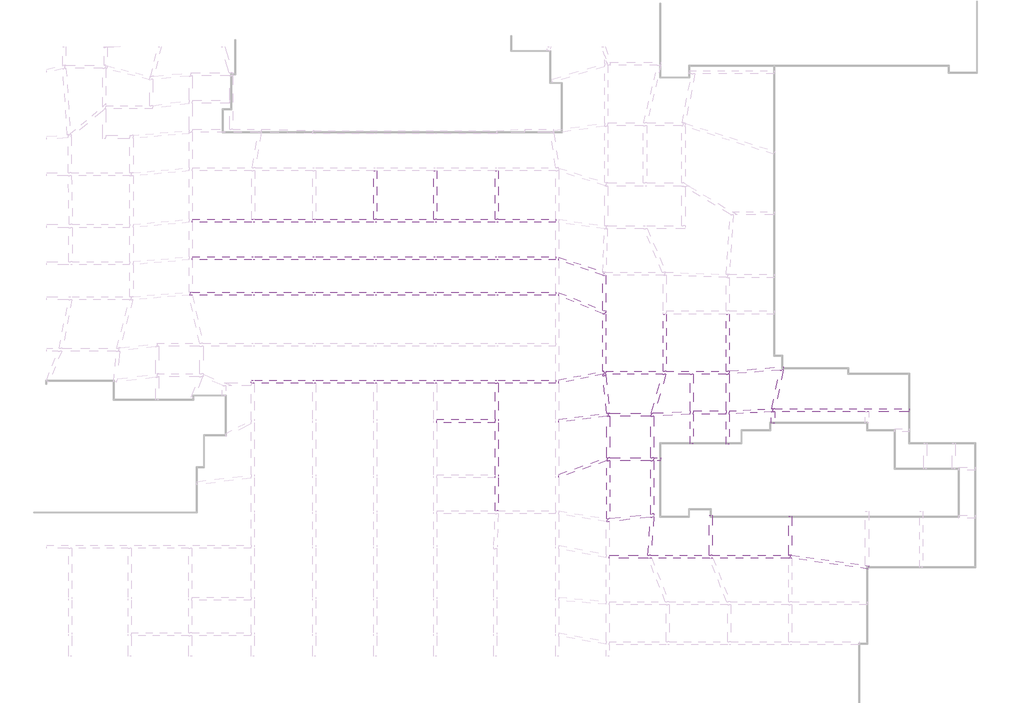
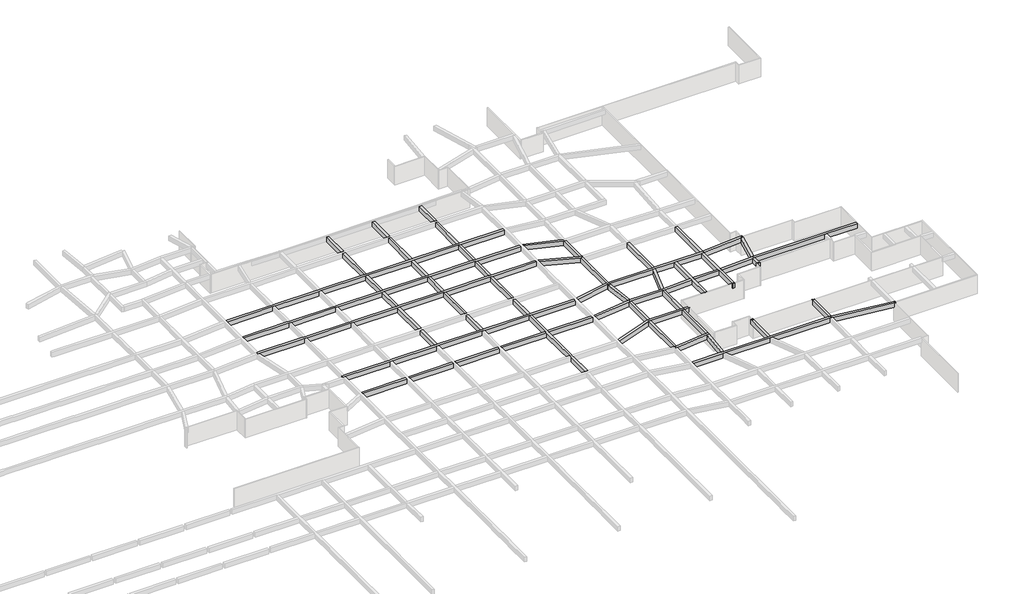
# One storey, part 40 of 45: 43 beams.
"""IFC4 building model written with IfcOpenShell, lengths in millimetres."""

from ifc_helpers import new_model, si_unit, frame, origin, place, context, project, spatial, polyline, outline, extrude, faceted_brep, element, save

model = new_model("IFC4")

# Units and contexts
model_context = context("Model", 3, world=origin())
ifc_project = project(units=[si_unit("LENGTHUNIT", "METRE", prefix="MILLI")], contexts=[model_context])

# Site, building, storey
site = spatial("IfcSite", under=ifc_project)
building = spatial("IfcBuilding", under=site)
storey = spatial("IfcBuildingStorey", under=building, Name="户型图", Elevation=0.0)

# Beams
placement = place(None, origin())
element("IfcBeam", 1, ObjectType="混凝土 - 矩形梁 : KL_beam", at=placement, inside=storey, context=model_context, shape_type="Brep", body=[
    faceted_brep([(24442.7166646, 44499.769125, 3300.0), (24442.7166646, 44899.769125, 3300.0), (17069.3873949, 44899.769125, 3300.0), (16669.3873949, 44899.769125, 3300.0), (9169.3873949, 44899.769125, 3300.0), (8769.3873949, 44899.769125, 3300.0), (1471.7652295, 44899.769125, 3300.0), (1071.7652295, 44899.769125, 3300.0), (-6328.2347705, 44899.769125, 3300.0), (-6728.2347705, 44899.769125, 3300.0), (-14137.8475592, 44899.769125, 3300.0), (-14537.8475592, 44899.769125, 3300.0), (-22164.0859234, 44899.769125, 3300.0), (-22164.0859234, 44499.769125, 3300.0), (-14537.8475592, 44499.769125, 3300.0), (-14137.8475592, 44499.769125, 3300.0), (-6728.2347705, 44499.769125, 3300.0), (-6328.2347705, 44499.769125, 3300.0), (1071.7652295, 44499.769125, 3300.0), (1471.7652295, 44499.769125, 3300.0), (8769.3873949, 44499.769125, 3300.0), (9169.3873949, 44499.769125, 3300.0), (16669.3873949, 44499.769125, 3300.0), (17069.3873949, 44499.769125, 3300.0), (24442.7166646, 44499.769125, 2500.0), (-22164.0859234, 44499.769125, 2500.0), (-14537.8475592, 44499.769125, 2500.0), (-14137.8475592, 44499.769125, 2500.0), (-6728.2347705, 44499.769125, 2500.0), (-6328.2347705, 44499.769125, 2500.0), (1071.7652295, 44499.769125, 2500.0), (1471.7652295, 44499.769125, 2500.0), (8769.3873949, 44499.769125, 2500.0), (9169.3873949, 44499.769125, 2500.0), (16669.3873949, 44499.769125, 2500.0), (17069.3873949, 44499.769125, 2500.0), (24442.7166646, 44899.769125, 2500.0), (-22164.0859234, 44899.769125, 2500.0), (-14537.8475592, 44899.769125, 2500.0), (-14137.8475592, 44899.769125, 2500.0), (-6728.2347705, 44899.769125, 2500.0), (-6328.2347705, 44899.769125, 2500.0), (1071.7652295, 44899.769125, 2500.0), (1471.7652295, 44899.769125, 2500.0), (8769.3873949, 44899.769125, 2500.0), (9169.3873949, 44899.769125, 2500.0), (16669.3873949, 44899.769125, 2500.0), (17069.3873949, 44899.769125, 2500.0)], [[[0, 1, 2, 3, 4, 5, 6, 7, 8, 9, 10, 11, 12, 13, 14, 15, 16, 17, 18, 19, 20, 21, 22, 23]], [[24, 0, 23, 22, 21, 20, 19, 18, 17, 16, 15, 14, 13, 25, 26, 27, 28, 29, 30, 31, 32, 33, 34, 35]], [[36, 24, 35, 34, 33, 32, 31, 30, 29, 28, 27, 26, 25, 37, 38, 39, 40, 41, 42, 43, 44, 45, 46, 47]], [[1, 36, 47, 46, 45, 44, 43, 42, 41, 40, 39, 38, 37, 12, 11, 10, 9, 8, 7, 6, 5, 4, 3, 2]], [[1, 0, 24, 36]], [[13, 12, 37, 25]]]),
])
element("IfcBeam", 2, ObjectType="混凝土 - 矩形梁 : KL_beam", at=placement, inside=storey, context=model_context, shape_type="Brep", body=[
    faceted_brep([(24442.7166646, 39701.2747355, 3300.0), (24442.7166646, 40101.2747355, 3300.0), (17069.3873949, 40101.2747355, 3300.0), (16669.3873949, 40101.2747355, 3300.0), (9169.3873949, 40101.2747355, 3300.0), (8769.3873949, 40101.2747355, 3300.0), (1471.7652295, 40101.2747355, 3300.0), (1071.7652295, 40101.2747355, 3300.0), (-6328.2347705, 40101.2747355, 3300.0), (-6728.2347705, 40101.2747355, 3300.0), (-14137.8475592, 40101.2747355, 3300.0), (-14537.8475592, 40101.2747355, 3300.0), (-22164.0859234, 40101.2747355, 3300.0), (-22164.0859234, 39701.2747355, 3300.0), (-14537.8475592, 39701.2747355, 3300.0), (-14137.8475592, 39701.2747355, 3300.0), (-6728.2347705, 39701.2747355, 3300.0), (-6328.2347705, 39701.2747355, 3300.0), (1071.7652295, 39701.2747355, 3300.0), (1471.7652295, 39701.2747355, 3300.0), (8769.3873949, 39701.2747355, 3300.0), (9169.3873949, 39701.2747355, 3300.0), (16669.3873949, 39701.2747355, 3300.0), (17069.3873949, 39701.2747355, 3300.0), (24442.7166646, 39701.2747355, 2500.0), (-22164.0859234, 39701.2747355, 2500.0), (-14537.8475592, 39701.2747355, 2500.0), (-14137.8475592, 39701.2747355, 2500.0), (-6728.2347705, 39701.2747355, 2500.0), (-6328.2347705, 39701.2747355, 2500.0), (1071.7652295, 39701.2747355, 2500.0), (1471.7652295, 39701.2747355, 2500.0), (8769.3873949, 39701.2747355, 2500.0), (9169.3873949, 39701.2747355, 2500.0), (16669.3873949, 39701.2747355, 2500.0), (17069.3873949, 39701.2747355, 2500.0), (24442.7166646, 40101.2747355, 2500.0), (-22164.0859234, 40101.2747355, 2500.0), (-14537.8475592, 40101.2747355, 2500.0), (-14137.8475592, 40101.2747355, 2500.0), (-6728.2347705, 40101.2747355, 2500.0), (-6328.2347705, 40101.2747355, 2500.0), (1071.7652295, 40101.2747355, 2500.0), (1471.7652295, 40101.2747355, 2500.0), (8769.3873949, 40101.2747355, 2500.0), (9169.3873949, 40101.2747355, 2500.0), (16669.3873949, 40101.2747355, 2500.0), (17069.3873949, 40101.2747355, 2500.0)], [[[0, 1, 2, 3, 4, 5, 6, 7, 8, 9, 10, 11, 12, 13, 14, 15, 16, 17, 18, 19, 20, 21, 22, 23]], [[24, 0, 23, 22, 21, 20, 19, 18, 17, 16, 15, 14, 13, 25, 26, 27, 28, 29, 30, 31, 32, 33, 34, 35]], [[36, 24, 35, 34, 33, 32, 31, 30, 29, 28, 27, 26, 25, 37, 38, 39, 40, 41, 42, 43, 44, 45, 46, 47]], [[1, 36, 47, 46, 45, 44, 43, 42, 41, 40, 39, 38, 37, 12, 11, 10, 9, 8, 7, 6, 5, 4, 3, 2]], [[1, 0, 24, 36]], [[13, 12, 37, 25]]]),
])
element("IfcBeam", 3, ObjectType="混凝土 - 矩形梁 : KL_beam", at=placement, inside=storey, context=model_context, shape_type="Brep", body=[
    faceted_brep([(-22423.5665565, 35573.301237, 3300.0), (-22407.6688706, 35173.301237, 3300.0), (-22167.3046288, 35173.301237, 3300.0), (-14537.8475592, 35173.301237, 3300.0), (-14137.8475592, 35173.301237, 3300.0), (-6728.2347705, 35173.301237, 3300.0), (-6328.2347705, 35173.301237, 3300.0), (1071.7652295, 35173.301237, 3300.0), (1471.7652295, 35173.301237, 3300.0), (8769.3873949, 35173.301237, 3300.0), (9169.3873949, 35173.301237, 3300.0), (16669.3873949, 35173.301237, 3300.0), (17069.3873949, 35173.301237, 3300.0), (24442.7166646, 35173.301237, 3300.0), (24442.7166646, 35573.301237, 3300.0), (17069.3873949, 35573.301237, 3300.0), (16669.3873949, 35573.301237, 3300.0), (9169.3873949, 35573.301237, 3300.0), (8769.3873949, 35573.301237, 3300.0), (1471.7652295, 35573.301237, 3300.0), (1071.7652295, 35573.301237, 3300.0), (-6328.2347705, 35573.301237, 3300.0), (-6728.2347705, 35573.301237, 3300.0), (-14137.8475592, 35573.301237, 3300.0), (-14537.8475592, 35573.301237, 3300.0), (-22164.0859234, 35573.301237, 3300.0), (-22407.6688706, 35173.301237, 2500.0), (-22167.3046288, 35173.301237, 2500.0), (-14537.8475592, 35173.301237, 2500.0), (-14137.8475592, 35173.301237, 2500.0), (-6728.2347705, 35173.301237, 2500.0), (-6328.2347705, 35173.301237, 2500.0), (1071.7652295, 35173.301237, 2500.0), (1471.7652295, 35173.301237, 2500.0), (8769.3873949, 35173.301237, 2500.0), (9169.3873949, 35173.301237, 2500.0), (16669.3873949, 35173.301237, 2500.0), (17069.3873949, 35173.301237, 2500.0), (24442.7166646, 35173.301237, 2500.0), (-22423.5665565, 35573.301237, 2500.0), (-22164.0859234, 35573.301237, 2500.0), (-14537.8475592, 35573.301237, 2500.0), (-14137.8475592, 35573.301237, 2500.0), (-6728.2347705, 35573.301237, 2500.0), (-6328.2347705, 35573.301237, 2500.0), (1071.7652295, 35573.301237, 2500.0), (1471.7652295, 35573.301237, 2500.0), (8769.3873949, 35573.301237, 2500.0), (9169.3873949, 35573.301237, 2500.0), (16669.3873949, 35573.301237, 2500.0), (17069.3873949, 35573.301237, 2500.0), (24442.7166646, 35573.301237, 2500.0)], [[[0, 1, 2, 3, 4, 5, 6, 7, 8, 9, 10, 11, 12, 13, 14, 15, 16, 17, 18, 19, 20, 21, 22, 23, 24, 25]], [[1, 26, 27, 28, 29, 30, 31, 32, 33, 34, 35, 36, 37, 38, 13, 12, 11, 10, 9, 8, 7, 6, 5, 4, 3, 2]], [[26, 39, 40, 41, 42, 43, 44, 45, 46, 47, 48, 49, 50, 51, 38, 37, 36, 35, 34, 33, 32, 31, 30, 29, 28, 27]], [[39, 0, 25, 24, 23, 22, 21, 20, 19, 18, 17, 16, 15, 14, 51, 50, 49, 48, 47, 46, 45, 44, 43, 42, 41, 40]], [[14, 13, 38, 51]], [[0, 39, 26, 1]]]),
])
element("IfcBeam", 4, ObjectType="混凝土 - 矩形梁 : KL_beam", at=placement, inside=storey, context=model_context, shape_type="Brep", body=[
    faceted_brep([(-14628.2347705, 24268.127427, 3300.0), (-14628.2347705, 23923.6357489, 3300.0), (-14628.2347705, 23868.127427, 3300.0), (-14228.2347705, 23868.127427, 3300.0), (-6728.2347705, 23868.127427, 3300.0), (-6328.2347705, 23868.127427, 3300.0), (1071.7652295, 23868.127427, 3300.0), (1471.7652295, 23868.127427, 3300.0), (8769.3873949, 23868.127427, 3300.0), (9169.3873949, 23868.127427, 3300.0), (16669.3873949, 23868.127427, 3300.0), (17069.3873949, 23868.127427, 3300.0), (24442.7166646, 23868.127427, 3300.0), (24442.7166646, 24268.127427, 3300.0), (17069.3873949, 24268.127427, 3300.0), (16669.3873949, 24268.127427, 3300.0), (9169.3873949, 24268.127427, 3300.0), (8769.3873949, 24268.127427, 3300.0), (1471.7652295, 24268.127427, 3300.0), (1071.7652295, 24268.127427, 3300.0), (-6328.2347705, 24268.127427, 3300.0), (-6728.2347705, 24268.127427, 3300.0), (-14137.8475592, 24268.127427, 3300.0), (-14537.8475592, 24268.127427, 3300.0), (-14628.2347705, 23868.127427, 2500.0), (-14228.2347705, 23868.127427, 2500.0), (-6728.2347705, 23868.127427, 2500.0), (-6328.2347705, 23868.127427, 2500.0), (1071.7652295, 23868.127427, 2500.0), (1471.7652295, 23868.127427, 2500.0), (8769.3873949, 23868.127427, 2500.0), (9169.3873949, 23868.127427, 2500.0), (16669.3873949, 23868.127427, 2500.0), (17069.3873949, 23868.127427, 2500.0), (24442.7166646, 23868.127427, 2500.0), (-14628.2347705, 23923.6357489, 2500.0), (-14628.2347705, 24268.127427, 2500.0), (-14537.8475592, 24268.127427, 2500.0), (-14137.8475592, 24268.127427, 2500.0), (-6728.2347705, 24268.127427, 2500.0), (-6328.2347705, 24268.127427, 2500.0), (1071.7652295, 24268.127427, 2500.0), (1471.7652295, 24268.127427, 2500.0), (8769.3873949, 24268.127427, 2500.0), (9169.3873949, 24268.127427, 2500.0), (16669.3873949, 24268.127427, 2500.0), (17069.3873949, 24268.127427, 2500.0), (24442.7166646, 24268.127427, 2500.0)], [[[0, 1, 2, 3, 4, 5, 6, 7, 8, 9, 10, 11, 12, 13, 14, 15, 16, 17, 18, 19, 20, 21, 22, 23]], [[2, 24, 25, 26, 27, 28, 29, 30, 31, 32, 33, 34, 12, 11, 10, 9, 8, 7, 6, 5, 4, 3]], [[24, 35, 36, 37, 38, 39, 40, 41, 42, 43, 44, 45, 46, 47, 34, 33, 32, 31, 30, 29, 28, 27, 26, 25]], [[36, 0, 23, 22, 21, 20, 19, 18, 17, 16, 15, 14, 13, 47, 46, 45, 44, 43, 42, 41, 40, 39, 38, 37]], [[2, 1, 0, 36, 35, 24]], [[13, 12, 34, 47]]]),
])
element("IfcBeam", 5, ObjectType="混凝土 - 矩形梁 : KL_beam", at=placement, inside=storey, context=model_context, shape_type="Brep", body=[
    faceted_brep([(17069.3873949, 23868.127427, 3300.0), (16669.3873949, 23868.127427, 3300.0), (16669.3873949, 19231.9876735, 3300.0), (16669.3873949, 18831.9876735, 3300.0), (16669.3873949, 12131.9876735, 3300.0), (16669.3873949, 11731.9876735, 3300.0), (16669.3873949, 7519.5822838, 3300.0), (17069.3873949, 7519.5822838, 3300.0), (17069.3873949, 11731.9876735, 3300.0), (17069.3873949, 12131.9876735, 3300.0), (17069.3873949, 18831.9876735, 3300.0), (17069.3873949, 19231.9876735, 3300.0), (16669.3873949, 23868.127427, 2500.0), (16669.3873949, 19231.9876735, 2500.0), (16669.3873949, 18831.9876735, 2500.0), (16669.3873949, 12131.9876735, 2500.0), (16669.3873949, 11731.9876735, 2500.0), (16669.3873949, 7519.5822838, 2500.0), (17069.3873949, 23868.127427, 2500.0), (17069.3873949, 19231.9876735, 2500.0), (17069.3873949, 18831.9876735, 2500.0), (17069.3873949, 12131.9876735, 2500.0), (17069.3873949, 11731.9876735, 2500.0), (17069.3873949, 7519.5822838, 2500.0)], [[[0, 1, 2, 3, 4, 5, 6, 7, 8, 9, 10, 11]], [[1, 12, 13, 14, 15, 16, 17, 6, 5, 4, 3, 2]], [[12, 18, 19, 20, 21, 22, 23, 17, 16, 15, 14, 13]], [[18, 0, 11, 10, 9, 8, 7, 23, 22, 21, 20, 19]], [[1, 0, 18, 12]], [[7, 6, 17, 23]]]),
])
element("IfcBeam", 6, ObjectType="混凝土 - 矩形梁 : KL_beam", at=placement, inside=storey, context=model_context, shape_type="SweptSolid", body=[
    extrude(outline(polyline([(1471.7652295, 24268.127427), (1071.7652295, 24268.127427), (1071.7652295, 28584.9161885), (1471.7652295, 28584.9161885), (1471.7652295, 24268.127427)])), frame((0.0, 0.0, 2500.0), z_axis=(0.0, 0.0, 1.0), x_axis=(1.0, 0.0, 0.0)), (0.0, 0.0, 1.0), 800.0),
    extrude(outline(polyline([(1071.7652295, 55873.039671), (1471.7652295, 55873.039671), (1471.7652295, 51521.1695582), (1071.7652295, 51521.1695582), (1071.7652295, 55873.039671)])), frame((0.0, 0.0, 2500.0), z_axis=(0.0, 0.0, 1.0), x_axis=(1.0, 0.0, 0.0)), (0.0, 0.0, 1.0), 800.0),
    extrude(outline(polyline([(1071.7652295, 51121.1695582), (1471.7652295, 51121.1695582), (1471.7652295, 44899.769125), (1071.7652295, 44899.769125), (1071.7652295, 51121.1695582)])), frame((0.0, 0.0, 2500.0), z_axis=(0.0, 0.0, 1.0), x_axis=(1.0, 0.0, 0.0)), (0.0, 0.0, 1.0), 800.0),
    extrude(outline(polyline([(1071.7652295, 44499.769125), (1471.7652295, 44499.769125), (1471.7652295, 40101.2747355), (1071.7652295, 40101.2747355), (1071.7652295, 44499.769125)])), frame((0.0, 0.0, 2500.0), z_axis=(0.0, 0.0, 1.0), x_axis=(1.0, 0.0, 0.0)), (0.0, 0.0, 1.0), 800.0),
    extrude(outline(polyline([(1071.7652295, 39701.2747355), (1471.7652295, 39701.2747355), (1471.7652295, 35573.301237), (1071.7652295, 35573.301237), (1071.7652295, 39701.2747355)])), frame((0.0, 0.0, 2500.0), z_axis=(0.0, 0.0, 1.0), x_axis=(1.0, 0.0, 0.0)), (0.0, 0.0, 1.0), 800.0),
    extrude(outline(polyline([(1071.7652295, 35173.301237), (1471.7652295, 35173.301237), (1471.7652295, 28984.9161885), (1071.7652295, 28984.9161885), (1071.7652295, 35173.301237)])), frame((0.0, 0.0, 2500.0), z_axis=(0.0, 0.0, 1.0), x_axis=(1.0, 0.0, 0.0)), (0.0, 0.0, 1.0), 800.0),
])
element("IfcBeam", 7, ObjectType="混凝土 - 矩形梁 : KL_beam", at=placement, inside=storey, context=model_context, shape_type="SweptSolid", body=[
    extrude(outline(polyline([(9169.3873949, 24268.127427), (8769.3873949, 24268.127427), (8769.3873949, 28584.9161885), (9169.3873949, 28584.9161885), (9169.3873949, 24268.127427)])), frame((0.0, 0.0, 2500.0), z_axis=(0.0, 0.0, 1.0), x_axis=(1.0, 0.0, 0.0)), (0.0, 0.0, 1.0), 800.0),
    extrude(outline(polyline([(8769.3873949, 55873.039671), (9169.3873949, 55873.039671), (9169.3873949, 51521.1695582), (8769.3873949, 51521.1695582), (8769.3873949, 55873.039671)])), frame((0.0, 0.0, 2500.0), z_axis=(0.0, 0.0, 1.0), x_axis=(1.0, 0.0, 0.0)), (0.0, 0.0, 1.0), 800.0),
    extrude(outline(polyline([(8769.3873949, 51121.1695582), (9169.3873949, 51121.1695582), (9169.3873949, 44899.769125), (8769.3873949, 44899.769125), (8769.3873949, 51121.1695582)])), frame((0.0, 0.0, 2500.0), z_axis=(0.0, 0.0, 1.0), x_axis=(1.0, 0.0, 0.0)), (0.0, 0.0, 1.0), 800.0),
    extrude(outline(polyline([(8769.3873949, 44499.769125), (9169.3873949, 44499.769125), (9169.3873949, 40101.2747355), (8769.3873949, 40101.2747355), (8769.3873949, 44499.769125)])), frame((0.0, 0.0, 2500.0), z_axis=(0.0, 0.0, 1.0), x_axis=(1.0, 0.0, 0.0)), (0.0, 0.0, 1.0), 800.0),
    extrude(outline(polyline([(8769.3873949, 39701.2747355), (9169.3873949, 39701.2747355), (9169.3873949, 35573.301237), (8769.3873949, 35573.301237), (8769.3873949, 39701.2747355)])), frame((0.0, 0.0, 2500.0), z_axis=(0.0, 0.0, 1.0), x_axis=(1.0, 0.0, 0.0)), (0.0, 0.0, 1.0), 800.0),
    extrude(outline(polyline([(8769.3873949, 35173.301237), (9169.3873949, 35173.301237), (9169.3873949, 28984.9161885), (8769.3873949, 28984.9161885), (8769.3873949, 35173.301237)])), frame((0.0, 0.0, 2500.0), z_axis=(0.0, 0.0, 1.0), x_axis=(1.0, 0.0, 0.0)), (0.0, 0.0, 1.0), 800.0),
])
element("IfcBeam", 8, ObjectType="混凝土 - 矩形梁 : KL_beam", at=placement, inside=storey, context=model_context, shape_type="SweptSolid", body=[
    extrude(outline(polyline([(16866.5611963, 55873.039671), (17069.3873949, 55883.6693417), (17069.3873949, 51521.1695582), (16669.3873949, 51521.1695582), (16669.3873949, 55873.039671), (16866.5611963, 55873.039671)])), frame((0.0, 0.0, 2500.0), z_axis=(0.0, 0.0, 1.0), x_axis=(1.0, 0.0, 0.0)), (0.0, 0.0, 1.0), 800.0),
    extrude(outline(polyline([(17069.3873949, 24268.127427), (16669.3873949, 24268.127427), (16669.3873949, 28584.9161885), (17069.3873949, 28584.9161885), (17069.3873949, 24268.127427)])), frame((0.0, 0.0, 2500.0), z_axis=(0.0, 0.0, 1.0), x_axis=(1.0, 0.0, 0.0)), (0.0, 0.0, 1.0), 800.0),
    extrude(outline(polyline([(16669.3873949, 51121.1695582), (17069.3873949, 51121.1695582), (17069.3873949, 44899.769125), (16669.3873949, 44899.769125), (16669.3873949, 51121.1695582)])), frame((0.0, 0.0, 2500.0), z_axis=(0.0, 0.0, 1.0), x_axis=(1.0, 0.0, 0.0)), (0.0, 0.0, 1.0), 800.0),
    extrude(outline(polyline([(16669.3873949, 44499.769125), (17069.3873949, 44499.769125), (17069.3873949, 40101.2747355), (16669.3873949, 40101.2747355), (16669.3873949, 44499.769125)])), frame((0.0, 0.0, 2500.0), z_axis=(0.0, 0.0, 1.0), x_axis=(1.0, 0.0, 0.0)), (0.0, 0.0, 1.0), 800.0),
    extrude(outline(polyline([(16669.3873949, 39701.2747355), (17069.3873949, 39701.2747355), (17069.3873949, 35573.301237), (16669.3873949, 35573.301237), (16669.3873949, 39701.2747355)])), frame((0.0, 0.0, 2500.0), z_axis=(0.0, 0.0, 1.0), x_axis=(1.0, 0.0, 0.0)), (0.0, 0.0, 1.0), 800.0),
    extrude(outline(polyline([(16669.3873949, 35173.301237), (17069.3873949, 35173.301237), (17069.3873949, 28984.9161885), (16669.3873949, 28984.9161885), (16669.3873949, 35173.301237)])), frame((0.0, 0.0, 2500.0), z_axis=(0.0, 0.0, 1.0), x_axis=(1.0, 0.0, 0.0)), (0.0, 0.0, 1.0), 800.0),
])
element("IfcBeam", 9, ObjectType="混凝土 - 矩形梁 : KL_beam", at=placement, inside=storey, context=model_context, shape_type="Brep", body=[
    faceted_brep([(30576.4538412, 37715.3996909, 3300.0), (30641.276919, 38115.3996909, 3300.0), (30478.0045918, 38169.7460466, 3300.0), (24842.7166646, 40045.4917239, 3300.0), (24842.7166646, 39623.9149013, 3300.0), (30469.2445302, 37751.0850728, 3300.0), (30641.276919, 38115.3996909, 2500.0), (30478.0045918, 38169.7460466, 2500.0), (24842.7166646, 40045.4917239, 2500.0), (30576.4538412, 37715.3996909, 2500.0), (30469.2445302, 37751.0850728, 2500.0), (24842.7166646, 39623.9149013, 2500.0)], [[[0, 1, 2, 3, 4, 5]], [[1, 6, 7, 8, 3, 2]], [[6, 9, 10, 11, 8, 7]], [[9, 0, 5, 4, 11, 10]], [[0, 9, 6, 1]], [[4, 3, 8, 11]]]),
])
element("IfcBeam", 10, ObjectType="混凝土 - 矩形梁 : KL_beam", at=placement, inside=storey, context=model_context, shape_type="Brep", body=[
    faceted_brep([(30719.4018928, 32702.3865413, 3300.0), (30869.2445302, 33073.2600831, 3300.0), (30469.2445302, 33234.8705735, 3300.0), (24842.7166646, 35508.1353916, 3300.0), (24842.7166646, 35076.7214945, 3300.0), (30469.2445302, 32803.4566764, 3300.0), (30719.4018928, 32702.3865413, 2500.0), (24842.7166646, 35076.7214945, 2500.0), (30469.2445302, 32803.4566764, 2500.0), (30869.2445302, 33073.2600831, 2500.0), (24842.7166646, 35508.1353916, 2500.0), (30469.2445302, 33234.8705735, 2500.0)], [[[0, 1, 2, 3, 4, 5]], [[6, 0, 5, 4, 7, 8]], [[9, 6, 8, 7, 10, 11]], [[1, 9, 11, 10, 3, 2]], [[4, 3, 10, 7]], [[1, 0, 6, 9]]]),
])
element("IfcBeam", 11, ObjectType="混凝土 - 矩形梁 : KL_beam", at=placement, inside=storey, context=model_context, shape_type="Brep", body=[
    faceted_brep([(30469.2445302, 33234.8705735, 3300.0), (30869.2445302, 33073.2600831, 3300.0), (30869.2445302, 33138.1514859, 3300.0), (30869.2445302, 37715.3996909, 3300.0), (30576.4538412, 37715.3996909, 3300.0), (30469.2445302, 37751.0850728, 3300.0), (30869.2445302, 33073.2600831, 2500.0), (30869.2445302, 33138.1514859, 2500.0), (30869.2445302, 37715.3996909, 2500.0), (30469.2445302, 33234.8705735, 2500.0), (30469.2445302, 37751.0850728, 2500.0), (30576.4538412, 37715.3996909, 2500.0)], [[[0, 1, 2, 3, 4, 5]], [[1, 6, 7, 8, 3, 2]], [[6, 9, 10, 11, 8, 7]], [[9, 0, 5, 10]], [[1, 0, 9, 6]], [[4, 3, 8, 11]], [[5, 4, 11, 10]]]),
])
element("IfcBeam", 12, ObjectType="混凝土 - 矩形梁 : KL_beam", at=placement, inside=storey, context=model_context, shape_type="Brep", body=[
    faceted_brep([(30591.7520122, 25428.338566, 3300.0), (30668.0756103, 25035.6876927, 3300.0), (30668.0756103, 25035.6876927, 2500.0), (30591.7520122, 25428.338566, 2500.0), (30469.2445302, 25404.5255238, 3300.0), (24842.7166646, 24310.8392979, 3300.0), (24842.7166646, 23903.3526199, 3300.0), (30469.2445302, 24997.0388458, 3300.0), (24842.7166646, 23903.3526199, 2500.0), (30469.2445302, 24997.0388458, 2500.0), (24842.7166646, 24310.8392979, 2500.0), (30469.2445302, 25404.5255238, 2500.0)], [[[0, 1, 2, 3]], [[1, 0, 4, 5, 6, 7]], [[2, 1, 7, 6, 8, 9]], [[3, 2, 9, 8, 10, 11]], [[0, 3, 11, 10, 5, 4]], [[6, 5, 10, 8]]]),
])
element("IfcBeam", 13, ObjectType="混凝土 - 矩形梁 : KL_beam", at=placement, inside=storey, context=model_context, shape_type="Brep", body=[
    faceted_brep([(46703.931079, 25032.0622988, 3300.0), (46703.931079, 25047.0116053, 3300.0), (46703.931079, 25432.0622988, 3300.0), (46303.931079, 25432.0622988, 3300.0), (38608.8653801, 25432.0622988, 3300.0), (38208.8653801, 25432.0622988, 3300.0), (30869.2445302, 25432.0622988, 3300.0), (30869.2445302, 25032.0622988, 3300.0), (38141.8774421, 25032.0622988, 3300.0), (38558.6848825, 25032.0622988, 3300.0), (41699.4783436, 25032.0622988, 3300.0), (42099.4783436, 25032.0622988, 3300.0), (46303.931079, 25032.0622988, 3300.0), (46703.931079, 25032.0622988, 2500.0), (30869.2445302, 25032.0622988, 2500.0), (38141.8774421, 25032.0622988, 2500.0), (38558.6848825, 25032.0622988, 2500.0), (41699.4783436, 25032.0622988, 2500.0), (42099.4783436, 25032.0622988, 2500.0), (46303.931079, 25032.0622988, 2500.0), (46703.931079, 25432.0622988, 2500.0), (46703.931079, 25047.0116053, 2500.0), (30869.2445302, 25432.0622988, 2500.0), (38208.8653801, 25432.0622988, 2500.0), (38608.8653801, 25432.0622988, 2500.0), (46303.931079, 25432.0622988, 2500.0)], [[[0, 1, 2, 3, 4, 5, 6, 7, 8, 9, 10, 11, 12]], [[13, 0, 12, 11, 10, 9, 8, 7, 14, 15, 16, 17, 18, 19]], [[20, 21, 13, 19, 18, 17, 16, 15, 14, 22, 23, 24, 25]], [[2, 20, 25, 24, 23, 22, 6, 5, 4, 3]], [[2, 1, 0, 13, 21, 20]], [[7, 6, 22, 14]]]),
])
element("IfcBeam", 14, ObjectType="混凝土 - 矩形梁 : KL_beam", at=placement, inside=storey, context=model_context, shape_type="Brep", body=[
    faceted_brep([(31205.7537894, 19636.32534, 3300.0), (31181.2887414, 20036.32534, 3300.0), (30974.2160413, 20010.9000095, 3300.0), (24842.7166646, 19258.0465508, 3300.0), (24842.7166646, 18855.0426206, 3300.0), (30993.5212654, 19610.2664627, 3300.0), (31205.7537894, 19636.32534, 2500.0), (24842.7166646, 18855.0426206, 2500.0), (30993.5212654, 19610.2664627, 2500.0), (31181.2887414, 20036.32534, 2500.0), (24842.7166646, 19258.0465508, 2500.0), (30974.2160413, 20010.9000095, 2500.0)], [[[0, 1, 2, 3, 4, 5]], [[6, 0, 5, 4, 7, 8]], [[9, 6, 8, 7, 10, 11]], [[1, 9, 11, 10, 3, 2]], [[4, 3, 10, 7]], [[1, 0, 6, 9]]]),
])
element("IfcBeam", 15, ObjectType="混凝土 - 矩形梁 : KL_beam", at=placement, inside=storey, context=model_context, shape_type="Brep", body=[
    faceted_brep([(36688.2840811, 20036.32534, 3300.0), (36678.520732, 20036.32534, 3300.0), (31373.7349949, 20036.32534, 3300.0), (31181.2887414, 20036.32534, 3300.0), (31205.7537894, 19636.32534, 3300.0), (31393.5212654, 19636.32534, 3300.0), (36630.442154, 19636.32534, 3300.0), (36698.7584497, 19636.32534, 3300.0), (31205.7537894, 19636.32534, 2500.0), (31393.5212654, 19636.32534, 2500.0), (36630.442154, 19636.32534, 2500.0), (36698.7584497, 19636.32534, 2500.0), (31181.2887414, 20036.32534, 2500.0), (31373.7349949, 20036.32534, 2500.0), (36678.520732, 20036.32534, 2500.0), (36688.2840811, 20036.32534, 2500.0)], [[[0, 1, 2, 3, 4, 5, 6, 7]], [[7, 6, 5, 4, 8, 9, 10, 11]], [[11, 10, 9, 8, 12, 13, 14, 15]], [[3, 2, 1, 0, 15, 14, 13, 12]], [[3, 12, 8, 4]], [[0, 7, 11, 15]]]),
])
element("IfcBeam", 16, ObjectType="混凝土 - 矩形梁 : KL_beam", at=placement, inside=storey, context=model_context, shape_type="Brep", body=[
    faceted_brep([(36688.2840811, 20036.32534, 3300.0), (36698.7584497, 19636.32534, 3300.0), (37030.442154, 19653.7081464, 3300.0), (41699.4783436, 19898.4019645, 3300.0), (41699.4783436, 20298.9509029, 3300.0), (37101.6742672, 20057.9902017, 3300.0), (36698.7584497, 19636.32534, 2500.0), (37030.442154, 19653.7081464, 2500.0), (41699.4783436, 19898.4019645, 2500.0), (36688.2840811, 20036.32534, 2500.0), (37101.6742672, 20057.9902017, 2500.0), (41699.4783436, 20298.9509029, 2500.0)], [[[0, 1, 2, 3, 4, 5]], [[1, 6, 7, 8, 3, 2]], [[6, 9, 10, 11, 8, 7]], [[9, 0, 5, 4, 11, 10]], [[0, 9, 6, 1]], [[4, 3, 8, 11]]]),
])
element("IfcBeam", 17, ObjectType="混凝土 - 矩形梁 : KL_beam", at=placement, inside=storey, context=model_context, shape_type="SweptSolid", body=[
    extrude(outline(polyline([(42099.4783436, 19913.7059081), (42099.4783436, 20313.7059081), (46303.931079, 20313.7059081), (46303.931079, 19913.7059081), (42099.4783436, 19913.7059081)])), frame((0.0, 0.0, 2500.0), z_axis=(0.0, 0.0, 1.0), x_axis=(1.0, 0.0, 0.0)), (0.0, 0.0, 1.0), 800.0),
])
element("IfcBeam", 18, ObjectType="混凝土 - 矩形梁 : KL_beam", at=placement, inside=storey, context=model_context, shape_type="SweptSolid", body=[
    extrude(outline(polyline([(24442.7166646, 19231.9876735), (24442.7166646, 18831.9876735), (17069.3873949, 18831.9876735), (17069.3873949, 19231.9876735), (24442.7166646, 19231.9876735)])), frame((0.0, 0.0, 2500.0), z_axis=(0.0, 0.0, 1.0), x_axis=(1.0, 0.0, 0.0)), (0.0, 0.0, 1.0), 800.0),
    extrude(outline(polyline([(-14228.2347705, 18831.9876735), (-14228.2347705, 19231.9876735), (-6728.2347705, 19231.9876735), (-6728.2347705, 18831.9876735), (-14228.2347705, 18831.9876735)])), frame((0.0, 0.0, 2500.0), z_axis=(0.0, 0.0, 1.0), x_axis=(1.0, 0.0, 0.0)), (0.0, 0.0, 1.0), 800.0),
    extrude(outline(polyline([(-6328.2347705, 18831.9876735), (-6328.2347705, 19231.9876735), (1071.7652295, 19231.9876735), (1071.7652295, 18831.9876735), (-6328.2347705, 18831.9876735)])), frame((0.0, 0.0, 2500.0), z_axis=(0.0, 0.0, 1.0), x_axis=(1.0, 0.0, 0.0)), (0.0, 0.0, 1.0), 800.0),
    extrude(outline(polyline([(1471.7652295, 18831.9876735), (1471.7652295, 19231.9876735), (8769.3873949, 19231.9876735), (8769.3873949, 18831.9876735), (1471.7652295, 18831.9876735)])), frame((0.0, 0.0, 2500.0), z_axis=(0.0, 0.0, 1.0), x_axis=(1.0, 0.0, 0.0)), (0.0, 0.0, 1.0), 800.0),
    extrude(outline(polyline([(9169.3873949, 18831.9876735), (9169.3873949, 19231.9876735), (16669.3873949, 19231.9876735), (16669.3873949, 18831.9876735), (9169.3873949, 18831.9876735)])), frame((0.0, 0.0, 2500.0), z_axis=(0.0, 0.0, 1.0), x_axis=(1.0, 0.0, 0.0)), (0.0, 0.0, 1.0), 800.0),
])
element("IfcBeam", 19, ObjectType="混凝土 - 矩形梁 : KL_beam", at=placement, inside=storey, context=model_context, shape_type="Brep", body=[
    faceted_brep([(31105.7115005, 13945.8511239, 3300.0), (31038.7744568, 14345.8511239, 3300.0), (30993.5212654, 14330.2692005, 3300.0), (24842.7166646, 12212.3773324, 3300.0), (24842.7166646, 11789.32906, 3300.0), (30993.5212654, 13907.220928, 3300.0), (31105.7115005, 13945.8511239, 2500.0), (24842.7166646, 11789.32906, 2500.0), (30993.5212654, 13907.220928, 2500.0), (31038.7744568, 14345.8511239, 2500.0), (24842.7166646, 12212.3773324, 2500.0), (30993.5212654, 14330.2692005, 2500.0)], [[[0, 1, 2, 3, 4, 5]], [[6, 0, 5, 4, 7, 8]], [[9, 6, 8, 7, 10, 11]], [[1, 9, 11, 10, 3, 2]], [[4, 3, 10, 7]], [[1, 0, 6, 9]]]),
])
element("IfcBeam", 20, ObjectType="混凝土 - 矩形梁 : KL_beam", at=placement, inside=storey, context=model_context, shape_type="Brep", body=[
    faceted_brep([(31038.7744568, 14345.8511239, 3300.0), (31105.7115005, 13945.8511239, 3300.0), (31393.5212654, 13945.8511239, 3300.0), (36630.442154, 13945.8511239, 3300.0), (37030.442154, 13945.8511239, 3300.0), (37030.442154, 14345.4372359, 3300.0), (37030.442154, 14345.8511239, 3300.0), (36630.442154, 14345.8511239, 3300.0), (31393.5212654, 14345.8511239, 3300.0), (31105.7115005, 13945.8511239, 2500.0), (31393.5212654, 13945.8511239, 2500.0), (36630.442154, 13945.8511239, 2500.0), (37030.442154, 13945.8511239, 2500.0), (31038.7744568, 14345.8511239, 2500.0), (31393.5212654, 14345.8511239, 2500.0), (36630.442154, 14345.8511239, 2500.0), (37030.442154, 14345.8511239, 2500.0), (37030.442154, 14345.4372359, 2500.0)], [[[0, 1, 2, 3, 4, 5, 6, 7, 8]], [[1, 9, 10, 11, 12, 4, 3, 2]], [[9, 13, 14, 15, 16, 17, 12, 11, 10]], [[13, 0, 8, 7, 6, 16, 15, 14]], [[0, 13, 9, 1]], [[6, 5, 4, 12, 17, 16]]]),
])
element("IfcBeam", 21, ObjectType="混凝土 - 矩形梁 : KL_beam", at=placement, inside=storey, context=model_context, shape_type="Brep", body=[
    faceted_brep([(31067.4957265, 6504.4149268, 3300.0), (31056.9345953, 6101.1015953, 3300.0), (31293.5212654, 6125.9678564, 3300.0), (36612.8120762, 6685.0478492, 3300.0), (37017.1957115, 6727.5502819, 3300.0), (37030.442154, 6728.9425391, 3300.0), (37030.442154, 7131.145851, 3300.0), (36630.442154, 7089.1041569, 3300.0), (31393.5212654, 6538.6815917, 3300.0), (31056.9345953, 6101.1015953, 2500.0), (31293.5212654, 6125.9678564, 2500.0), (36612.8120762, 6685.0478492, 2500.0), (37017.1957115, 6727.5502819, 2500.0), (37030.442154, 6728.9425391, 2500.0), (31067.4957265, 6504.4149268, 2500.0), (31393.5212654, 6538.6815917, 2500.0), (36630.442154, 7089.1041569, 2500.0), (37030.442154, 7131.145851, 2500.0)], [[[0, 1, 2, 3, 4, 5, 6, 7, 8]], [[1, 9, 10, 11, 12, 13, 5, 4, 3, 2]], [[9, 14, 15, 16, 17, 13, 12, 11, 10]], [[14, 0, 8, 7, 6, 17, 16, 15]], [[0, 14, 9, 1]], [[6, 5, 13, 17]]]),
])
element("IfcBeam", 22, ObjectType="混凝土 - 矩形梁 : KL_beam", at=placement, inside=storey, context=model_context, shape_type="Brep", body=[
    faceted_brep([(37030.442154, 13945.8511239, 3300.0), (36630.442154, 13945.8511239, 3300.0), (36630.442154, 7089.1041569, 3300.0), (37030.442154, 7131.145851, 3300.0), (37030.442154, 13945.4372359, 3300.0), (37030.442154, 13945.8511239, 2500.0), (37030.442154, 7131.145851, 2500.0), (37030.442154, 13945.4372359, 2500.0), (36630.442154, 13945.8511239, 2500.0), (36630.442154, 7089.1041569, 2500.0)], [[[0, 1, 2, 3, 4]], [[5, 0, 4, 3, 6, 7]], [[8, 5, 7, 6, 9]], [[1, 8, 9, 2]], [[1, 0, 5, 8]], [[3, 2, 9, 6]]]),
])
element("IfcBeam", 23, ObjectType="混凝土 - 矩形梁 : KL_beam", at=placement, inside=storey, context=model_context, shape_type="SweptSolid", body=[
    extrude(outline(polyline([(37030.442154, 14345.8511239), (36630.442154, 14345.8511239), (36630.442154, 19636.32534), (36698.7584497, 19636.32534), (37030.442154, 19653.7081464), (37030.442154, 14345.8511239)])), frame((0.0, 0.0, 2500.0), z_axis=(0.0, 0.0, 1.0), x_axis=(1.0, 0.0, 0.0)), (0.0, 0.0, 1.0), 800.0),
])
element("IfcBeam", 24, ObjectType="混凝土 - 矩形梁 : KL_beam", at=placement, inside=storey, context=model_context, shape_type="SweptSolid", body=[
    extrude(outline(polyline([(31181.2887414, 20036.32534), (30974.2160413, 20010.9000095), (30469.2445302, 24849.5366195), (30469.2445302, 24860.1514859), (30869.2445302, 24860.1514859), (30869.2445302, 24870.3525647), (31373.7349949, 20036.32534), (31181.2887414, 20036.32534)])), frame((0.0, 0.0, 2500.0), z_axis=(0.0, 0.0, 1.0), x_axis=(1.0, 0.0, 0.0)), (0.0, 0.0, 1.0), 800.0),
])
element("IfcBeam", 25, ObjectType="混凝土 - 矩形梁 : KL_beam", at=placement, inside=storey, context=model_context, shape_type="Brep", body=[
    faceted_brep([(31393.5212654, 19636.32534, 3300.0), (31205.7537894, 19636.32534, 3300.0), (31015.7423586, 19612.9948699, 3300.0), (30993.5212654, 19610.2664627, 3300.0), (30993.5212654, 14330.2692005, 3300.0), (31038.7744568, 14345.8511239, 3300.0), (31393.5212654, 14345.8511239, 3300.0), (30993.5212654, 19610.2664627, 2500.0), (30993.5212654, 14330.2692005, 2500.0), (31205.7537894, 19636.32534, 2500.0), (31393.5212654, 19636.32534, 2500.0), (31393.5212654, 14345.8511239, 2500.0), (31038.7744568, 14345.8511239, 2500.0), (31015.7423586, 19612.9948699, 2500.0)], [[[0, 1, 2, 3, 4, 5, 6]], [[3, 7, 8, 4]], [[9, 10, 11, 12, 8, 7, 13]], [[10, 0, 6, 11]], [[7, 3, 2, 1, 9, 13]], [[1, 0, 10, 9]], [[6, 5, 12, 11]], [[5, 4, 8, 12]]]),
])
element("IfcBeam", 26, ObjectType="混凝土 - 矩形梁 : KL_beam", at=placement, inside=storey, context=model_context, shape_type="SweptSolid", body=[
    extrude(outline(polyline([(31393.5212654, 6538.6815917), (31067.4957265, 6504.4149268), (30993.5212654, 6516.1313304), (30993.5212654, 13907.220928), (31105.7115005, 13945.8511239), (31393.5212654, 13945.8511239), (31393.5212654, 6538.6815917)])), frame((0.0, 0.0, 2500.0), z_axis=(0.0, 0.0, 1.0), x_axis=(1.0, 0.0, 0.0)), (0.0, 0.0, 1.0), 800.0),
])
element("IfcBeam", 27, ObjectType="混凝土 - 矩形梁 : KL_beam", at=placement, inside=storey, context=model_context, shape_type="Brep", body=[
    faceted_brep([(42099.4783436, 16132.0622988, 3300.0), (41699.4783436, 16132.0622988, 3300.0), (41699.4783436, 16132.0622988, 2500.0), (42099.4783436, 16132.0622988, 2500.0), (42099.4783436, 19913.7059081, 3300.0), (42099.4783436, 20313.7059081, 3300.0), (42099.4783436, 25032.0622988, 3300.0), (41699.4783436, 25032.0622988, 3300.0), (41699.4783436, 20298.9509029, 3300.0), (41699.4783436, 19898.4019645, 3300.0), (41699.4783436, 25032.0622988, 2500.0), (41699.4783436, 20298.9509029, 2500.0), (41699.4783436, 19898.4019645, 2500.0), (42099.4783436, 25032.0622988, 2500.0), (42099.4783436, 20313.7059081, 2500.0), (42099.4783436, 19913.7059081, 2500.0)], [[[0, 1, 2, 3]], [[1, 0, 4, 5, 6, 7, 8, 9]], [[2, 1, 9, 8, 7, 10, 11, 12]], [[3, 2, 12, 11, 10, 13, 14, 15]], [[0, 3, 15, 14, 13, 6, 5, 4]], [[7, 6, 13, 10]]]),
])
element("IfcBeam", 28, ObjectType="混凝土 - 矩形梁 : KL_beam", at=placement, inside=storey, context=model_context, shape_type="Brep", body=[
    faceted_brep([(38558.6848825, 25032.0622988, 3300.0), (38141.8774421, 25032.0622988, 3300.0), (36678.520732, 20036.32534, 3300.0), (36688.2840811, 20036.32534, 3300.0), (37030.442154, 20054.2570848, 3300.0), (37101.6742672, 20057.9902017, 3300.0), (38558.6848825, 25032.0622988, 2500.0), (37101.6742672, 20057.9902017, 2500.0), (38141.8774421, 25032.0622988, 2500.0), (37030.442154, 20054.2570848, 2500.0), (36688.2840811, 20036.32534, 2500.0), (36678.520732, 20036.32534, 2500.0)], [[[0, 1, 2, 3, 4, 5]], [[6, 0, 5, 7]], [[8, 6, 7, 9, 10, 11]], [[1, 8, 11, 2]], [[1, 0, 6, 8]], [[7, 5, 4, 3, 10, 9]], [[3, 2, 11, 10]]]),
])
element("IfcBeam", 29, ObjectType="混凝土 - 矩形梁 : KL_beam", at=placement, inside=storey, context=model_context, shape_type="SweptSolid", body=[
    extrude(outline(polyline([(38208.8653801, 32715.3996909), (38608.8653801, 32715.3996909), (38608.8653801, 25432.0622988), (38208.8653801, 25432.0622988), (38208.8653801, 32715.3996909)])), frame((0.0, 0.0, 2500.0), z_axis=(0.0, 0.0, 1.0), x_axis=(1.0, 0.0, 0.0)), (0.0, 0.0, 1.0), 800.0),
])
element("IfcBeam", 30, ObjectType="混凝土 - 矩形梁 : KL_beam", at=placement, inside=storey, context=model_context, shape_type="Brep", body=[
    faceted_brep([(30869.2445302, 24860.1514859, 3300.0), (30469.2445302, 24860.1514859, 3300.0), (30469.2445302, 24860.1514859, 2500.0), (30869.2445302, 24860.1514859, 2500.0), (30869.2445302, 24870.3525647, 3300.0), (30869.2445302, 25032.0622988, 3300.0), (30869.2445302, 25432.0622988, 3300.0), (30869.2445302, 32738.1514859, 3300.0), (30869.2445302, 33073.2600831, 3300.0), (30719.4018928, 32702.3865413, 3300.0), (30469.2445302, 32803.4566764, 3300.0), (30469.2445302, 25404.5255238, 3300.0), (30591.7520122, 25428.338566, 3300.0), (30668.0756103, 25035.6876927, 3300.0), (30469.2445302, 24997.0388458, 3300.0), (30469.2445302, 24997.0388458, 2500.0), (30668.0756103, 25035.6876927, 2500.0), (30591.7520122, 25428.338566, 2500.0), (30469.2445302, 25404.5255238, 2500.0), (30469.2445302, 32803.4566764, 2500.0), (30719.4018928, 32702.3865413, 2500.0), (30869.2445302, 33073.2600831, 2500.0), (30869.2445302, 32738.1514859, 2500.0), (30869.2445302, 25432.0622988, 2500.0), (30869.2445302, 25032.0622988, 2500.0), (30869.2445302, 24870.3525647, 2500.0)], [[[0, 1, 2, 3]], [[1, 0, 4, 5, 6, 7, 8, 9, 10, 11, 12, 13, 14]], [[2, 1, 14, 15]], [[3, 2, 15, 16, 17, 18, 19, 20, 21, 22, 23, 24, 25]], [[0, 3, 25, 24, 23, 22, 21, 8, 7, 6, 5, 4]], [[9, 20, 19, 10]], [[20, 9, 8, 21]], [[13, 16, 15, 14]], [[17, 12, 11, 18]], [[10, 19, 18, 11]], [[16, 13, 12, 17]]]),
])
element("IfcBeam", 31, ObjectType="混凝土 - 矩形梁 : KL_beam", at=placement, inside=storey, context=model_context, shape_type="Brep", body=[
    faceted_brep([(46303.931079, 25432.0622988, 3300.0), (46703.931079, 25432.0622988, 3300.0), (46703.931079, 25448.2148094, 3300.0), (46703.931079, 32738.1514859, 3300.0), (46303.931079, 32738.1514859, 3300.0), (46303.931079, 25432.0622988, 2500.0), (46303.931079, 32738.1514859, 2500.0), (46703.931079, 25432.0622988, 2500.0), (46703.931079, 32738.1514859, 2500.0), (46703.931079, 25448.2148094, 2500.0)], [[[0, 1, 2, 3, 4]], [[5, 0, 4, 6]], [[7, 5, 6, 8, 9]], [[1, 7, 9, 8, 3, 2]], [[1, 0, 5, 7]], [[4, 3, 8, 6]]]),
])
element("IfcBeam", 32, ObjectType="混凝土 - 矩形梁 : KL_beam", at=placement, inside=storey, context=model_context, shape_type="Brep", body=[
    faceted_brep([(54479.6593749, 1446.1972666, 3300.0), (54507.3831559, 1846.1972666, 3300.0), (54293.5212654, 1846.1972666, 3300.0), (44493.5212654, 1846.1972666, 3300.0), (44093.5212654, 1846.1972666, 3300.0), (36646.2186674, 1846.1972666, 3300.0), (36245.0651666, 1846.1972666, 3300.0), (31293.5212654, 1846.1972666, 3300.0), (31293.5212654, 1446.1972666, 3300.0), (36294.5011943, 1446.1972666, 3300.0), (36724.6875387, 1446.1972666, 3300.0), (44157.5803056, 1446.1972666, 3300.0), (44587.7666501, 1446.1972666, 3300.0), (54293.5212654, 1446.1972666, 3300.0), (54479.6593749, 1446.1972666, 2500.0), (31293.5212654, 1446.1972666, 2500.0), (36294.5011943, 1446.1972666, 2500.0), (36724.6875387, 1446.1972666, 2500.0), (44157.5803056, 1446.1972666, 2500.0), (44587.7666501, 1446.1972666, 2500.0), (54293.5212654, 1446.1972666, 2500.0), (54507.3831559, 1846.1972666, 2500.0), (31293.5212654, 1846.1972666, 2500.0), (36245.0651666, 1846.1972666, 2500.0), (36646.2186674, 1846.1972666, 2500.0), (44093.5212654, 1846.1972666, 2500.0), (44493.5212654, 1846.1972666, 2500.0), (54293.5212654, 1846.1972666, 2500.0)], [[[0, 1, 2, 3, 4, 5, 6, 7, 8, 9, 10, 11, 12, 13]], [[14, 0, 13, 12, 11, 10, 9, 8, 15, 16, 17, 18, 19, 20]], [[21, 14, 20, 19, 18, 17, 16, 15, 22, 23, 24, 25, 26, 27]], [[1, 21, 27, 26, 25, 24, 23, 22, 7, 6, 5, 4, 3, 2]], [[8, 7, 22, 15]], [[1, 0, 14, 21]]]),
])
element("IfcBeam", 33, ObjectType="混凝土 - 矩形梁 : KL_beam", at=placement, inside=storey, context=model_context, shape_type="Brep", body=[
    faceted_brep([(64559.4783436, 446.0608655, 3300.0), (64159.4783436, 501.7760721, 3300.0), (54693.5212654, 1820.2704585, 3300.0), (54507.3831559, 1846.1972666, 3300.0), (54479.6593749, 1446.1972666, 3300.0), (54693.5212654, 1416.408868, 3300.0), (64504.2958672, 49.8855327, 3300.0), (54479.6593749, 1446.1972666, 2500.0), (54693.5212654, 1416.408868, 2500.0), (64504.2958672, 49.8855327, 2500.0), (54507.3831559, 1846.1972666, 2500.0), (54693.5212654, 1820.2704585, 2500.0), (64159.4783436, 501.7760721, 2500.0), (64559.4783436, 446.0608655, 2500.0)], [[[0, 1, 2, 3, 4, 5, 6]], [[6, 5, 4, 7, 8, 9]], [[9, 8, 7, 10, 11, 12, 13]], [[3, 2, 1, 0, 13, 12, 11, 10]], [[3, 10, 7, 4]], [[0, 6, 9, 13]]]),
])
element("IfcBeam", 34, ObjectType="混凝土 - 矩形梁 : KL_beam", at=placement, inside=storey, context=model_context, shape_type="SweptSolid", body=[
    extrude(outline(polyline([(36646.2186674, 1846.1972666), (36245.0651666, 1846.1972666), (36612.8120762, 6685.0478492), (37017.1957115, 6727.5502819), (36646.2186674, 1846.1972666)])), frame((0.0, 0.0, 2500.0), z_axis=(0.0, 0.0, 1.0), x_axis=(1.0, 0.0, 0.0)), (0.0, 0.0, 1.0), 800.0),
])
element("IfcBeam", 35, ObjectType="混凝土 - 矩形梁 : KL_beam", at=placement, inside=storey, context=model_context, shape_type="SweptSolid", body=[
    extrude(outline(polyline([(44093.5212654, 6946.1972666), (44493.5212654, 6946.1972666), (44493.5212654, 1846.1972666), (44093.5212654, 1846.1972666), (44093.5212654, 6946.1972666)])), frame((0.0, 0.0, 2500.0), z_axis=(0.0, 0.0, 1.0), x_axis=(1.0, 0.0, 0.0)), (0.0, 0.0, 1.0), 800.0),
])
element("IfcBeam", 36, ObjectType="混凝土 - 矩形梁 : KL_beam", at=placement, inside=storey, context=model_context, shape_type="SweptSolid", body=[
    extrude(outline(polyline([(54293.5212654, 6845.4882174), (54693.5212654, 6845.4882174), (54693.5212654, 1820.2704585), (54507.3831559, 1846.1972666), (54293.5212654, 1846.1972666), (54293.5212654, 6845.4882174)])), frame((0.0, 0.0, 2500.0), z_axis=(0.0, 0.0, 1.0), x_axis=(1.0, 0.0, 0.0)), (0.0, 0.0, 1.0), 800.0),
])
element("IfcBeam", 37, ObjectType="混凝土 - 矩形梁 : KL_beam", at=placement, inside=storey, context=model_context, shape_type="Brep", body=[
    faceted_brep([(46703.931079, 16032.0622988, 3300.0), (46303.931079, 16032.0622988, 3300.0), (46303.931079, 16032.0622988, 2500.0), (46703.931079, 16032.0622988, 2500.0), (46703.931079, 19923.9248582, 3300.0), (46703.931079, 20324.4737966, 3300.0), (46703.931079, 25032.0622988, 3300.0), (46303.931079, 25032.0622988, 3300.0), (46303.931079, 20313.7059081, 3300.0), (46303.931079, 19913.7059081, 3300.0), (46303.931079, 25032.0622988, 2500.0), (46303.931079, 20313.7059081, 2500.0), (46303.931079, 19913.7059081, 2500.0), (46703.931079, 25032.0622988, 2500.0), (46703.931079, 20324.4737966, 2500.0), (46703.931079, 19923.9248582, 2500.0)], [[[0, 1, 2, 3]], [[1, 0, 4, 5, 6, 7, 8, 9]], [[2, 1, 9, 8, 7, 10, 11, 12]], [[3, 2, 12, 11, 10, 13, 14, 15]], [[0, 3, 15, 14, 13, 6, 5, 4]], [[7, 6, 13, 10]]]),
])
element("IfcBeam", 38, ObjectType="混凝土 - 矩形梁 : KL_beam", at=placement, inside=storey, context=model_context, shape_type="Brep", body=[
    faceted_brep([(53592.3593471, 25982.9036739, 3300.0), (46703.931079, 25448.2148094, 3300.0), (46703.931079, 25432.0622988, 3300.0), (46703.931079, 25047.0116053, 3300.0), (53206.953984, 25551.7847985, 3300.0), (53623.3147592, 25584.1032696, 3300.0), (46703.931079, 25047.0116053, 2500.0), (53206.953984, 25551.7847985, 2500.0), (53623.3147592, 25584.1032696, 2500.0), (46703.931079, 25432.0622988, 2500.0), (46703.931079, 25448.2148094, 2500.0), (53592.3593471, 25982.9036739, 2500.0)], [[[0, 1, 2, 3, 4, 5]], [[5, 4, 3, 6, 7, 8]], [[8, 7, 6, 9, 10, 11]], [[1, 0, 11, 10]], [[6, 3, 2, 1, 10, 9]], [[0, 5, 8, 11]]]),
])
element("IfcBeam", 39, ObjectType="混凝土 - 矩形梁 : KL_beam", at=placement, inside=storey, context=model_context, shape_type="Brep", body=[
    faceted_brep([(52300.9931971, 20217.2544543, 3300.0), (52290.5188285, 20617.2544543, 3300.0), (52132.7557771, 20608.9864431, 3300.0), (46703.931079, 20324.4737966, 3300.0), (46703.931079, 19923.9248582, 3300.0), (52095.7560128, 20206.4984293, 3300.0), (52300.9931971, 20217.2544543, 2500.0), (46703.9310789, 19923.9248582, 2500.0), (52095.7560128, 20206.4984293, 2500.0), (52290.5188285, 20617.2544543, 2500.0), (46703.931079, 20324.4737966, 2500.0), (52132.7557771, 20608.9864431, 2500.0)], [[[0, 1, 2, 3, 4, 5]], [[6, 0, 5, 4, 7, 8]], [[9, 6, 8, 7, 10, 11]], [[1, 9, 11, 10, 3, 2]], [[4, 3, 10, 7]], [[1, 0, 6, 9]]]),
])
element("IfcBeam", 40, ObjectType="混凝土 - 矩形梁 : KL_beam", at=placement, inside=storey, context=model_context, shape_type="Brep", body=[
    faceted_brep([(69759.1171782, 20617.2544543, 3300.0), (69759.1171782, 20217.2544543, 3300.0), (69759.1171782, 20217.2544543, 2500.0), (69759.1171782, 20617.2544543, 2500.0), (52543.8897639, 20617.2544543, 3300.0), (52290.5188285, 20617.2544543, 3300.0), (52300.9931971, 20217.2544543, 3300.0), (52495.7560128, 20217.2544543, 3300.0), (64159.4783436, 20217.2544543, 3300.0), (64559.4783436, 20217.2544543, 3300.0), (52300.9931971, 20217.2544543, 2500.0), (52495.7560128, 20217.2544543, 2500.0), (64159.4783436, 20217.2544543, 2500.0), (64559.4783436, 20217.2544543, 2500.0), (52290.5188285, 20617.2544543, 2500.0), (52543.8897639, 20617.2544543, 2500.0)], [[[0, 1, 2, 3]], [[1, 0, 4, 5, 6, 7, 8, 9]], [[2, 1, 9, 8, 7, 6, 10, 11, 12, 13]], [[3, 2, 13, 12, 11, 10, 14, 15]], [[0, 3, 15, 14, 5, 4]], [[5, 14, 10, 6]]]),
])
element("IfcBeam", 41, ObjectType="混凝土 - 矩形梁 : KL_beam", at=placement, inside=storey, context=model_context, shape_type="SweptSolid", body=[
    extrude(outline(polyline([(53206.953984, 25551.7847985), (53623.3147592, 25584.1032696), (52543.8897639, 20617.2544543), (52290.5188285, 20617.2544543), (52132.7557771, 20608.9864431), (53206.953984, 25551.7847985)])), frame((0.0, 0.0, 2500.0), z_axis=(0.0, 0.0, 1.0), x_axis=(1.0, 0.0, 0.0)), (0.0, 0.0, 1.0), 800.0),
])
element("IfcBeam", 42, ObjectType="混凝土 - 矩形梁 : KL_beam", at=placement, inside=storey, context=model_context, shape_type="Brep", body=[
    faceted_brep([(52495.7560128, 18717.2544543, 3300.0), (52095.7560128, 18717.2544543, 3300.0), (52095.7560128, 18717.2544543, 2500.0), (52495.7560128, 18717.2544543, 2500.0), (52495.7560128, 20217.2544543, 3300.0), (52456.9593954, 20217.2544543, 3300.0), (52300.9931971, 20217.2544543, 3300.0), (52095.7560128, 20206.4984293, 3300.0), (52095.7560128, 20206.4984293, 2500.0), (52300.9931971, 20217.2544543, 2500.0), (52456.9593954, 20217.2544543, 2500.0), (52495.7560128, 20217.2544543, 2500.0)], [[[0, 1, 2, 3]], [[1, 0, 4, 5, 6, 7]], [[2, 1, 7, 8]], [[3, 2, 8, 9, 10, 11]], [[0, 3, 11, 4]], [[7, 6, 9, 8]], [[4, 11, 10, 9, 6, 5]]]),
])
element("IfcBeam", 43, ObjectType="混凝土 - 矩形梁 : KL_beam", at=placement, inside=storey, context=model_context, shape_type="Brep", body=[
    faceted_brep([(37930.442154, 14345.4372359, 3300.0), (37930.442154, 13945.4372359, 3300.0), (37930.442154, 13945.4372359, 2500.0), (37930.442154, 14345.4372359, 2500.0), (37030.442154, 14345.4372359, 3300.0), (37030.442154, 13945.8511239, 3300.0), (37030.442154, 13945.4372359, 3300.0), (37030.442154, 13945.4372359, 2500.0), (37030.442154, 13945.8511239, 2500.0), (37030.442154, 14345.4372359, 2500.0)], [[[0, 1, 2, 3]], [[1, 0, 4, 5, 6]], [[2, 1, 6, 7]], [[3, 2, 7, 8, 9]], [[0, 3, 9, 4]], [[4, 9, 8, 7, 6, 5]]]),
])

save(model, "model.ifc")

# Revit data of these elements
# Type "混凝土 - 矩形梁 : KL_beam"
#   Length [instance default] = 1524 mm
#   b = 400 mm
#   h = 800 mm
#   Structural Material [instance default] = 混凝土 - 现场浇注混凝土
#   Assembly Code = ""
# Elements 1, 2, 3, 4, 5, 6, 7, 8, 9, 10, 11, 12, 13, 14, 15, 16, 17, 18, 19, 20, 21, 22, 23, 24, 25, 26, 27, 28, 29, 30, 31, 32, 33, 34, 35, 36, 37, 38, 39, 40, 41, 42, 43 (IfcBeam, "混凝土 - 矩形梁 : KL_beam")
#   Comments = ""
#   Structural Material = none
#   Phase Created = 新构造
# Materials
#   "混凝土 - 现场浇注混凝土": class "混凝土", colour RGB 192 192 192, transparency 0
